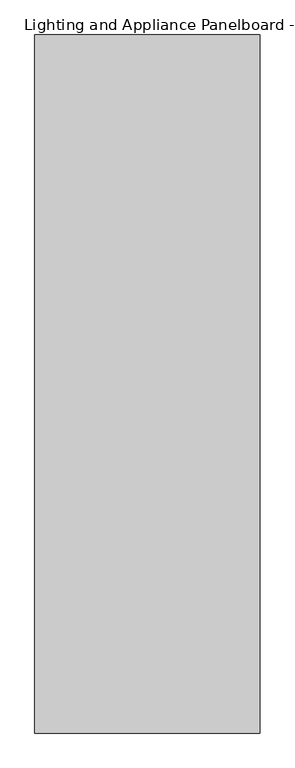
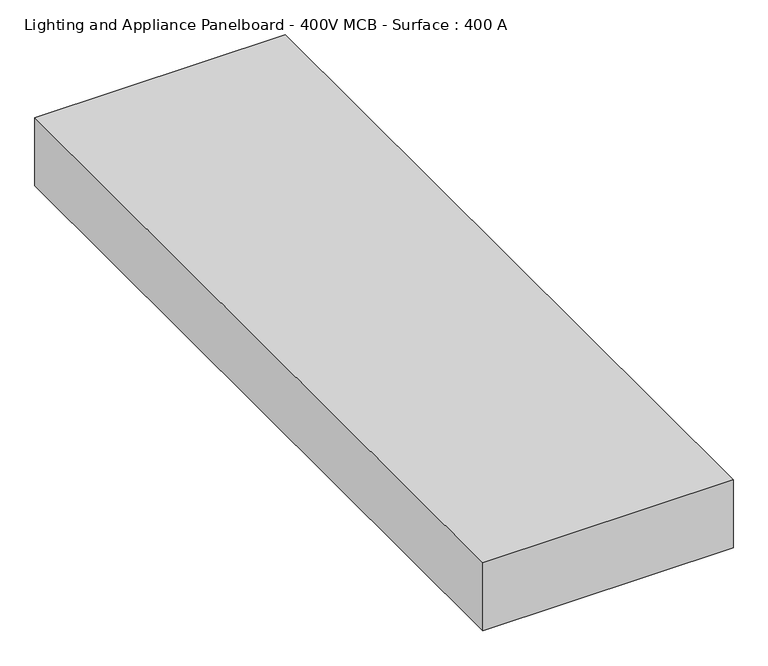
"""IFC4 building model written with IfcOpenShell, lengths in millimetres: proxy geometry, Lighting and Appliance Panelboard - 400V MCB - Surface : 400 A."""

from ifc_helpers import new_model, si_unit, origin, origin_with_axes, place, context, project, spatial, polyline, outline, extrude, source, transform, mapped, element, save


def lighting_and_appliance_panelboard_400v_mcb_surface_400_a_826206d9(model_context):
    return source(origin(), model_context, "Body", "SweptSolid", [
        extrude(outline(polyline([(254.0, -1574.8), (-254.0, -1574.8), (-254.0, 0.0), (254.0, 0.0), (254.0, -1574.8)])), origin_with_axes(), (0.0, 0.0, 1.0), 146.1),
    ])


if __name__ == "__main__":
    model = new_model("IFC4")
    model_context = context("Model", 3, world=origin())
    ifc_project = project(units=[si_unit("LENGTHUNIT", "METRE", prefix="MILLI")], contexts=[model_context])
    site = spatial("IfcSite", under=ifc_project)
    building = spatial("IfcBuilding", under=site)
    placement = place(None, origin())
    lighting_and_appliance_panelboard_400v_mcb_surface_400_a_shape = lighting_and_appliance_panelboard_400v_mcb_surface_400_a_826206d9(model_context)
    element("IfcBuildingElementProxy", 1, Name="Lighting and Appliance Panelboard - 400V MCB - Surface : 400 A", ObjectType="Lighting and Appliance Panelboard - 400V MCB - Surface : 400 A", at=placement, inside=building, context=model_context, shape_type="MappedRepresentation", body=[
        mapped(lighting_and_appliance_panelboard_400v_mcb_surface_400_a_shape, transform((0.0, 0.0, 0.0), x_axis=(1.0, 0.0, 0.0), y_axis=(0.0, 1.0, 0.0), z_axis=(0.0, 0.0, 1.0))),
    ])
    save(model, "model.ifc")

# Revit data of these elements
# Type "Lighting and Appliance Panelboard - 400V MCB - Surface : 400 A"
#   Type Mark = "Lighting and Appliance Panelboard - 400V MCB - Surface"
#   Classification.OmniClass.21.Number = "21-04 50 30 50"
#   Classification.MasterFormat.Description = "Wiring Devices"
#   Classification.OmniClass.22.Number = "22-26 27 26"
#   Classification.OmniClass.21.Description = "Wiring Devices"
#   Classification.UniFormat.II.Description = "Wiring Devices"
#   Classification.MasterFormat.Number = "26 27 26"
#   Classification.OmniClass.23.Number = "23-35 31 29"
#   Classification.OmniClass.22.Description = "Wiring Devices"
#   Classification.OmniClass.23.Description = "Switchboards"
#   Classification.UniFormat.II.Number = "D5030.50"
#   COBie.Type.CreatedBy = "info@mma.ie"
#   COBie.Type.CreatedOn = "2017-07-25T10:15:16"
#   COBie.Type.Name = "Lighting and Appliance Panelboard - 400V MCB - Surface"
#   COBie.Type.Category = "23-35 31 29 : Switchboards"
#   COBie.Type.Description = "Lighting and Appliance Panelboard - 400V MCB - Surface_400 A"
#   COBie.Type.AssetType = "Fixed"
#   COBie.Type.Manufacturer = ""
#   COBie.Type.ModelNumber = ""
#   Wattage = "400"
#   Voltage = "600"
#   built-in parameter 1140081 [instance default] = "Surface"
#   Keynote = "26 24 16.A"
#   built-in parameter 1140083 [instance default] = "Type 1"
#   COBie.Type.ReplacementCost = 0
#   Width = 508 mm
#   built-in parameter 1140082 [instance default] = 100 (stored number, unit not read)
#   built-in parameter 1140140 [instance default] = 400 (stored number, unit not read)
#   L.A.P. Width = 508 mm
#   L.A.P. Height = 1574.8 mm
#   L.A.P. Depth = 146.1 mm
#   Height [instance default] = 1574.8 mm
#   Depth = 146.1 mm
#   Default Elevation = 1200 mm
#   Ballast Wattage = 400 W
#   Ballast Voltage = 600 V
#   42 Circuit Height = 1727.2 mm
#   30 Circuit Height = 1574.8 mm
#   18 Circuit Height = 1574.8 mm
#   12 Circuit Height = 1574.8 mm
#   COBie.Type = yes
#   built-in parameter 1140142 [instance default] = -1
#   built-in parameter 1140079 [instance default] = 12
#   built-in parameter 1155100 [instance default] = -1
#   Load Classification = Other
